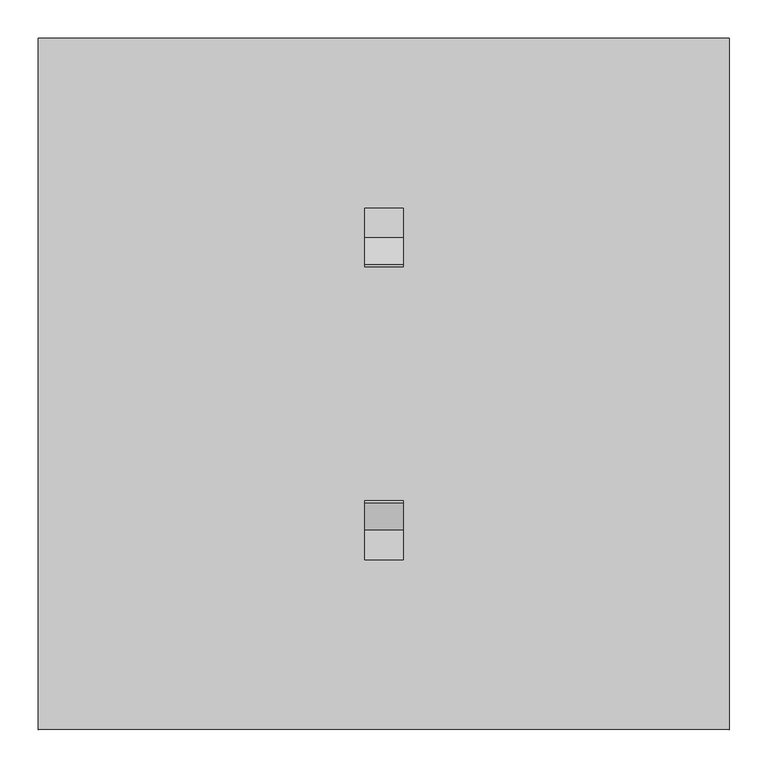
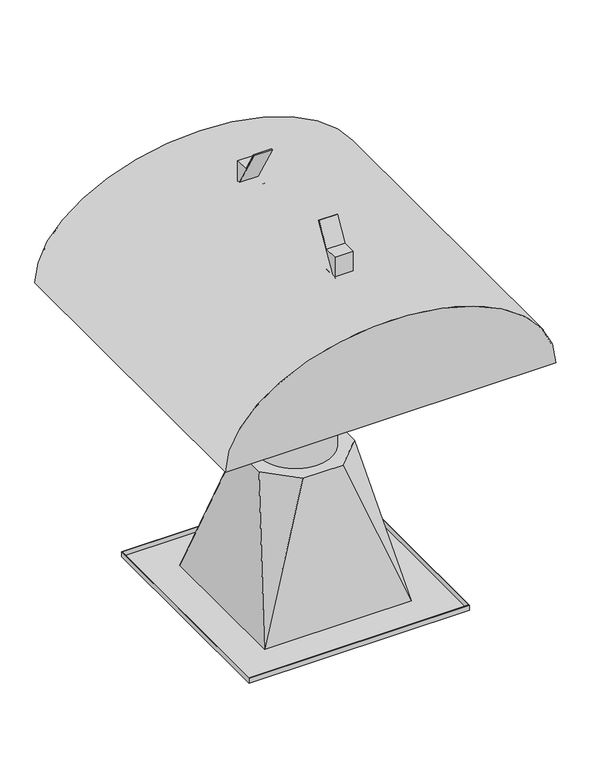
"""IFC4 building model written with IfcOpenShell, lengths in millimetres: proxy geometry, ВЕЗА_ВКОП : ВКОПО-040-Н-00."""

from ifc_helpers import new_model, si_unit, point, frame, frame_2d, origin, place, context, project, spatial, polyline, circle_curve, ellipse_curve, trimmed, segment, composite_curve, outline, extrude, faceted_brep, source, transform, mapped, element, save
from ifc_brep_helpers import plane_surface, cylinder_surface, revolved_surface, extruded_surface, advanced_brep


def mechanical_equipment_59a7846b(model_context):
    return source(origin(), model_context, "Body", "SolidModel", [
        extrude(outline(composite_curve([segment(trimmed(circle_curve(frame_2d((0.0, -15.0)), 15.0), [point((0.0, -30.0))], [point((0.0, 0.0))], False, "CARTESIAN"), True, "CONTINUOUS"), segment(trimmed(circle_curve(frame_2d((0.0, -15.0)), 15.0), [point((0.0, 0.0))], [point((0.0, -30.0))], False, "CARTESIAN"), True, "CONTINUOUS")], self_intersect=False), holes=[composite_curve([segment(trimmed(circle_curve(frame_2d((0.0, -15.0)), 8.0), [point((0.0, -23.0))], [point((0.0, -7.0))], True, "CARTESIAN"), True, "CONTINUOUS"), segment(trimmed(circle_curve(frame_2d((0.0, -15.0)), 8.0), [point((0.0, -7.0))], [point((0.0, -23.0))], True, "CARTESIAN"), True, "CONTINUOUS")], self_intersect=False)]), frame((119.501046, -59.3969696, 580.0), z_axis=(0.7071067811865491, 0.7071067811865459, 0.0), x_axis=(-0.7071067811865459, 0.7071067811865491, 0.0)), (0.0, 0.0, 1.0), 10.0),
        extrude(outline(composite_curve([segment(trimmed(circle_curve(frame_2d((0.0, -15.0)), 15.0), [point((0.0, -30.0))], [point((0.0, 0.0))], False, "CARTESIAN"), True, "CONTINUOUS"), segment(trimmed(circle_curve(frame_2d((0.0, -15.0)), 15.0), [point((0.0, 0.0))], [point((0.0, -30.0))], False, "CARTESIAN"), True, "CONTINUOUS")], self_intersect=False), holes=[composite_curve([segment(trimmed(circle_curve(frame_2d((0.0, -15.0)), 8.0), [point((0.0, -23.0))], [point((0.0, -7.0))], True, "CARTESIAN"), True, "CONTINUOUS"), segment(trimmed(circle_curve(frame_2d((0.0, -15.0)), 8.0), [point((0.0, -7.0))], [point((0.0, -23.0))], True, "CARTESIAN"), True, "CONTINUOUS")], self_intersect=False)]), frame((52.3259018, -126.5721138, 580.0), z_axis=(0.7071067811865491, 0.7071067811865459, 0.0), x_axis=(-0.7071067811865459, 0.7071067811865491, 0.0)), (0.0, 0.0, 1.0), 10.0),
        extrude(outline(composite_curve([segment(trimmed(circle_curve(frame_2d((89.4490078, -89.4490078)), 15.0), [point((100.0556095, -78.8424061))], [point((78.8424061, -100.0556095))], False, "CARTESIAN"), True, "CONTINUOUS"), segment(trimmed(circle_curve(frame_2d((89.4490078, -89.4490078)), 15.0), [point((78.8424061, -100.0556095))], [point((100.0556095, -78.8424061))], False, "CARTESIAN"), True, "CONTINUOUS")], self_intersect=False), holes=[composite_curve([segment(trimmed(circle_curve(frame_2d((89.4490078, -89.4490078)), 8.0), [point((95.1058621, -83.7921536))], [point((83.7921536, -95.1058621))], True, "CARTESIAN"), True, "CONTINUOUS"), segment(trimmed(circle_curve(frame_2d((89.4490078, -89.4490078)), 8.0), [point((83.7921536, -95.1058621))], [point((95.1058621, -83.7921536))], True, "CARTESIAN"), True, "CONTINUOUS")], self_intersect=False)]), frame((0.0, 0.0, 512.5), z_axis=(0.0, 0.0, 1.0), x_axis=(1.0, 0.0, 0.0)), (0.0, 0.0, 1.0), 10.0),
        extrude(outline(composite_curve([segment(trimmed(circle_curve(frame_2d((89.4490078, -89.4490078)), 15.0), [point((100.0556095, -78.8424061))], [point((78.8424061, -100.0556095))], False, "CARTESIAN"), True, "CONTINUOUS"), segment(trimmed(circle_curve(frame_2d((89.4490078, -89.4490078)), 15.0), [point((78.8424061, -100.0556095))], [point((100.0556095, -78.8424061))], False, "CARTESIAN"), True, "CONTINUOUS")], self_intersect=False), holes=[composite_curve([segment(trimmed(circle_curve(frame_2d((89.4490078, -89.4490078)), 8.0), [point((95.1058621, -83.7921536))], [point((83.7921536, -95.1058621))], True, "CARTESIAN"), True, "CONTINUOUS"), segment(trimmed(circle_curve(frame_2d((89.4490078, -89.4490078)), 8.0), [point((83.7921536, -95.1058621))], [point((95.1058621, -83.7921536))], True, "CARTESIAN"), True, "CONTINUOUS")], self_intersect=False)]), frame((0.0, 0.0, 607.5), z_axis=(0.0, 0.0, 1.0), x_axis=(1.0, 0.0, 0.0)), (0.0, 0.0, 1.0), 10.0),
        extrude(outline(polyline([(137.1787156, -77.0746391), (77.0746391, -137.1787156), (41.7193001, -101.8233765), (101.8233765, -41.7193001), (137.1787156, -77.0746391)])), frame((0.0, 0.0, 522.5), z_axis=(0.0, 0.0, 1.0), x_axis=(1.0, 0.0, 0.0)), (0.0, 0.0, 1.0), 85.0),
        extrude(outline(polyline([(190.7885358, 1086.3333333), (229.0846729, 1086.3333333), (229.0846729, 1030.0), (219.8766872, 1030.0), (152.3533268, 1146.953891), (154.9302621, 1148.4416853), (190.7885358, 1086.3333333)])), frame((-25.0, 0.0, 0.0), z_axis=(1.0, 0.0, 0.0), x_axis=(0.0, 1.0, 0.0)), (0.0, 0.0, 1.0), 50.0),
        extrude(outline(polyline([(189.0846729, 730.0), (189.0846729, 1028.0), (229.0846729, 1028.0), (448.0, 928.6666667), (448.0, 829.3333333), (229.0846729, 730.0), (189.0846729, 730.0)]), holes=[polyline([(194.0846729, 735.0), (228.0033477, 735.0), (443.0, 832.5552256), (443.0, 925.4447744), (228.0033477, 1023.0), (194.0846729, 1023.0), (194.0846729, 735.0)])]), frame((-25.0, 0.0, 0.0), z_axis=(1.0, 0.0, 0.0), x_axis=(0.0, 1.0, 0.0)), (0.0, 0.0, 1.0), 50.0),
        extrude(outline(polyline([(-190.7885358, 1086.3333333), (-154.9302621, 1148.4416853), (-152.3533268, 1146.953891), (-219.8766872, 1030.0), (-229.0846729, 1030.0), (-229.0846729, 1086.3333333), (-190.7885358, 1086.3333333)])), frame((-25.0, 0.0, 0.0), z_axis=(1.0, 0.0, 0.0), x_axis=(0.0, 1.0, 0.0)), (0.0, 0.0, 1.0), 50.0),
        extrude(outline(polyline([(-189.0846729, 730.0), (-229.0846729, 730.0), (-448.0, 829.3333333), (-448.0, 928.6666667), (-229.0846729, 1028.0), (-189.0846729, 1028.0), (-189.0846729, 730.0)]), holes=[polyline([(-194.0846729, 735.0), (-194.0846729, 1023.0), (-228.0033477, 1023.0), (-443.0, 925.4447744), (-443.0, 832.5552256), (-228.0033477, 735.0), (-194.0846729, 735.0)])]), frame((-25.0, 0.0, 0.0), z_axis=(1.0, 0.0, 0.0), x_axis=(0.0, 1.0, 0.0)), (0.0, 0.0, 1.0), 50.0),
        faceted_brep([(130.0, 53.8477631, 400.0), (53.8477631, 130.0, 400.0), (-53.8477631, 130.0, 400.0), (-130.0, 53.8477631, 400.0), (-130.0, -53.8477631, 400.0), (-53.8477631, -130.0, 400.0), (53.8477631, -130.0, 400.0), (130.0, -53.8477631, 400.0), (200.0, 200.0, 0.0), (200.0, -200.0, 0.0), (-200.0, -200.0, 0.0), (-200.0, 200.0, 0.0)], [[[0, 1, 2, 3, 4, 5, 6, 7]], [[8, 9, 10, 11]], [[1, 0, 8]], [[8, 11, 2, 1]], [[3, 2, 11]], [[11, 10, 4, 3]], [[5, 4, 10]], [[10, 9, 6, 5]], [[7, 6, 9]], [[9, 8, 0, 7]]]),
        advanced_brep(
        [(450.0, -450.0, 750.0), (-450.0, -450.0, 750.0), (450.0, 450.0, 750.0), (-450.0, 450.0, 750.0), (-448.0, -448.0, 750.0), (448.0, -448.0, 750.0), (448.0, 448.0, 750.0), (-448.0, 448.0, 750.0)],
        [
            (0, 1, ellipse_curve(frame((0.0, -450.0, 750.0), z_axis=(0.0, -1.0, 0.0), x_axis=(-1.0, 0.0, 0.0)), 450.0, 280.0)),
            (1, 0),
            (2, 3),
            (3, 2, ellipse_curve(frame((0.0, 450.0, 750.0), z_axis=(0.0, 1.0, 0.0), x_axis=(-1.0, 0.0, 0.0)), 450.0, 280.0)),
            (0, 2),
            (3, 1),
            (4, 5),
            (5, 6),
            (6, 7),
            (7, 4),
            (4, 5, ellipse_curve(frame((0.0, -448.0, 750.0), z_axis=(0.0, 1.0, 0.0), x_axis=(-1.0, 0.0, 0.0)), 448.0, 278.0)),
            (6, 7, ellipse_curve(frame((0.0, 448.0, 750.0), z_axis=(0.0, -1.0, 0.0), x_axis=(-1.0, 0.0, 0.0)), 448.0, 278.0)),
        ],
        [
            plane_surface(frame((-450.0, -450.0, 750.0), z_axis=(0.0, -1.0, 0.0), x_axis=(0.0, 0.0, -1.0))),
            plane_surface(frame((-450.0, 450.0, 750.0), z_axis=(0.0, 1.0, 0.0), x_axis=(0.0, 0.0, 1.0))),
            extruded_surface(trimmed(ellipse_curve(frame((0.0, 1350.0, 750.0), z_axis=(0.0, -1.0, 0.0), x_axis=(-1.0, 0.0, 0.0)), 450.0, 280.0), [point((450.0, 1350.0, 750.0))], [point((-450.0, 1350.0, 750.0))], True, "CARTESIAN"), (0.0, -900.0, 0.0), 900.0),
            plane_surface(frame((-450.0, -450.0, 750.0), z_axis=(0.0, 0.0, -1.0), x_axis=(0.0, 1.0, 0.0))),
            plane_surface(frame((-448.0, -448.0, 750.0), z_axis=(0.0, 1.0, 0.0), x_axis=(0.0, 0.0, -1.0))),
            plane_surface(frame((-448.0, 448.0, 750.0), z_axis=(0.0, -1.0, 0.0), x_axis=(0.0, 0.0, 1.0))),
            extruded_surface(trimmed(ellipse_curve(frame((0.0, 448.0, 750.0), z_axis=(0.0, -1.0, 0.0), x_axis=(-1.0, 0.0, 0.0)), 448.0, 278.0), [point((448.0, 448.0, 750.0))], [point((-448.0, 448.0, 750.0))], True, "CARTESIAN"), (0.0, 896.0, 0.0), 896.0),
        ],
        [
            (0, [[1, 2]]),
            (1, [[3, 4]]),
            (2, [[-1, 5, -4, 6]]),
            (3, [[-2, -6, -3, -5], [7, 8, 9, 10]]),
            (4, [[11, -7]]),
            (5, [[12, -9]]),
            (6, [[-11, -10, -12, -8]]),
        ],
    ),
        advanced_brep(
        [(130.0, 0.0, 730.0), (-130.0, 0.0, 730.0), (-45.0, 0.0, 730.0), (45.0, 0.0, 730.0), (100.0, 0.0, 686.5584821), (-100.0, 0.0, 686.5584821), (100.0, 0.0, 400.0), (-100.0, 0.0, 400.0), (0.0, 0.0, 400.0), (-45.0, 0.0, 750.0), (45.0, 0.0, 750.0)],
        [
            (0, 1, circle_curve(frame((0.0, 0.0, 730.0), z_axis=(0.0, 0.0, 1.0), x_axis=(-1.0, 0.0, 0.0)), 130.0)),
            (1, 2),
            (2, 3, circle_curve(frame((0.0, 0.0, 730.0), z_axis=(0.0, 0.0, -1.0), x_axis=(-1.0, 0.0, 0.0)), 45.0)),
            (3, 0),
            (1, 0, circle_curve(frame((0.0, 0.0, 730.0), z_axis=(0.0, 0.0, 1.0), x_axis=(-1.0, 0.0, 0.0)), 130.0)),
            (3, 2, circle_curve(frame((0.0, 0.0, 730.0), z_axis=(0.0, 0.0, -1.0), x_axis=(-1.0, 0.0, 0.0)), 45.0)),
            (0, 4, circle_curve(frame((151.2012649, 0.0, 683.2792411), z_axis=(0.0, -1.0, 0.0), x_axis=(-1.0, 0.0, 0.0)), 51.3061687)),
            (4, 5, circle_curve(frame((0.0, 0.0, 686.5584821), z_axis=(0.0, 0.0, 1.0), x_axis=(-1.0, 0.0, 0.0)), 100.0)),
            (5, 1, circle_curve(frame((-151.2012649, 0.0, 683.2792411), z_axis=(0.0, -1.0, 0.0), x_axis=(1.0, 0.0, 0.0)), 51.3061687)),
            (5, 4, circle_curve(frame((0.0, 0.0, 686.5584821), z_axis=(0.0, 0.0, 1.0), x_axis=(-1.0, 0.0, 0.0)), 100.0)),
            (4, 6),
            (6, 7, circle_curve(frame((0.0, 0.0, 400.0), z_axis=(0.0, 0.0, 1.0), x_axis=(-1.0, 0.0, 0.0)), 100.0)),
            (7, 5),
            (7, 6, circle_curve(frame((0.0, 0.0, 400.0), z_axis=(0.0, 0.0, 1.0), x_axis=(-1.0, 0.0, 0.0)), 100.0)),
            (6, 8),
            (8, 7),
            (2, 9),
            (9, 10, circle_curve(frame((0.0, 0.0, 750.0), z_axis=(0.0, 0.0, -1.0), x_axis=(-1.0, 0.0, 0.0)), 45.0)),
            (10, 3),
            (10, 9, circle_curve(frame((0.0, 0.0, 750.0), z_axis=(0.0, 0.0, -1.0), x_axis=(-1.0, 0.0, 0.0)), 45.0)),
        ],
        [
            plane_surface(frame((0.0, 0.0, 730.0), z_axis=(0.0, 0.0, 1.0), x_axis=(-1.0, 0.0, 0.0))),
            revolved_surface(trimmed(ellipse_curve(frame((-151.2012649, 0.0, 683.2792411), z_axis=(0.0, 1.0, 0.0), x_axis=(1.0, 0.0, 0.0)), 51.3061687, 51.3061687), [point((-130.0, 0.0, 730.0))], [point((-100.0, 0.0, 686.5584821))], True, "CARTESIAN"), (0.0, 0.0, 710.0), (0.0, 0.0, -1.0)),
            cylinder_surface(frame((0.0, 0.0, 710.0), z_axis=(0.0, 0.0, -1.0), x_axis=(-1.0, 0.0, 0.0)), 100.0),
            plane_surface(frame((0.0, 0.0, 400.0), z_axis=(0.0, 0.0, -1.0), x_axis=(-1.0, 0.0, 0.0))),
            cylinder_surface(frame((0.0, 0.0, 710.0), z_axis=(0.0, 0.0, -1.0), x_axis=(-1.0, 0.0, 0.0)), 45.0),
            plane_surface(frame((-448.0, -448.0, 750.0), z_axis=(0.0, 0.0, 1.0), x_axis=(0.0, 1.0, 0.0))),
        ],
        [
            (0, [[1, 2, 3, 4]]),
            (0, [[-2, 5, -4, 6]]),
            (1, [[-1, 7, 8, 9]]),
            (1, [[-5, -9, 10, -7]]),
            (2, [[-8, 11, 12, 13]]),
            (2, [[-10, -13, 14, -11]]),
            (3, [[-12, 15, 16]]),
            (3, [[-14, -16, -15]]),
            (4, [[-3, 17, 18, 19]]),
            (4, [[-6, -19, 20, -17]]),
            (5, [[-18, -20]]),
        ],
    ),
        faceted_brep([(-200.0, -200.0, 0.0), (-200.0, -200.0, 1.5), (200.0, -200.0, 1.5), (200.0, -200.0, 0.0), (-300.0, -300.0, 15.0), (-300.0, -300.0, 0.0), (300.0, -300.0, 0.0), (300.0, -300.0, 15.0), (-298.5, -298.5, 1.5), (-298.5, -298.5, 15.0), (298.5, -298.5, 15.0), (298.5, -298.5, 1.5), (200.0, 200.0, 1.5), (200.0, 200.0, 0.0), (300.0, 300.0, 0.0), (300.0, 300.0, 15.0), (298.5, 298.5, 15.0), (298.5, 298.5, 1.5), (-200.0, 200.0, 1.5), (-200.0, 200.0, 0.0), (-300.0, 300.0, 0.0), (-300.0, 300.0, 15.0), (-298.5, 298.5, 15.0), (-298.5, 298.5, 1.5)], [[[0, 1, 2, 3]], [[4, 5, 6, 7]], [[8, 9, 10, 11]], [[3, 2, 12, 13]], [[7, 6, 14, 15]], [[11, 10, 16, 17]], [[13, 12, 18, 19]], [[15, 14, 20, 21]], [[17, 16, 22, 23]], [[19, 18, 1, 0]], [[5, 20, 14, 6], [3, 13, 19, 0]], [[21, 20, 5, 4]], [[7, 15, 21, 4], [9, 22, 16, 10]], [[23, 22, 9, 8]], [[11, 17, 23, 8], [1, 18, 12, 2]]]),
    ])


if __name__ == "__main__":
    model = new_model("IFC4")
    model_context = context("Model", 3, world=origin())
    ifc_project = project(units=[si_unit("LENGTHUNIT", "METRE", prefix="MILLI")], contexts=[model_context])
    site = spatial("IfcSite", under=ifc_project)
    building = spatial("IfcBuilding", under=site)
    placement = place(None, origin())
    mechanical_equipment_shape = mechanical_equipment_59a7846b(model_context)
    element("IfcBuildingElementProxy", 1, Name="ВЕЗА_ВКОП : ВКОПО-040-Н-00", ObjectType="ВЕЗА_ВКОП : ВКОПО-040-Н-00", at=placement, inside=building, context=model_context, shape_type="MappedRepresentation", body=[
        mapped(mechanical_equipment_shape, transform((0.0, 0.0, 0.0), x_axis=(1.0, 0.0, 0.0), y_axis=(0.0, 1.0, 0.0), z_axis=(0.0, 0.0, 1.0))),
    ])
    save(model, "model.ifc")

# Revit data of these elements
# Type "ВЕЗА_ВКОП : ВКОПО-040-Н-00"
#   Таблица_ВКОП = "ВКОП"
#   Класс энергоэффективности электродвигателя = "IE2"
#   ВЕЗА_Контакты = "bim@veza.ru"
#   ВЕЗА_Классификатор = "79001"
#   URL = "http://www.veza.ru/upload/iblock/0e3/%D0%92%D0%9A%D0%9E%D0%9F%20%D0%B0%D0%B2%D0%B3%D1%83%D1%81%D1%82%202019%20%D1%80%D0%B5%D0%B4%D0%B0%D0%BA%D1%82%20270919-1.pdf"
#   ADSK_Примечание = ""
#   ADSK_Позиция = "1"
#   ADSK_Наименование краткое = "ВКОП"
#   ADSK_Наименование = "Агрегат крышный ВКОП 0 типоразмер 040; общепромышленного исполнения; номинальная мощность Nnon=1,1 кВт, число полюсов 2; климатическое исполение УХЛ1"
#   ADSK_Марка = "ВКОПО-040-Н-00110/2-УХЛ1 ТУ 4861-152-40149153-2010"
#   ADSK_Комплект [instance default] = ""
#   ADSK_Код изделия = ""
#   ADSK_Завод-изготовитель = "ООО \"Веза\", Россия, Москва, ИНН 505001001, info@veza.ru"
#   ADSK_Единица измерения = "компл."
#   ADSK_Дата изменения = "23.03.2020"
#   ADSK_Группирование = ""
#   ADSK_Версия семейства = "Версия 1"
#   ADSK_Версия Revit = "Revit2018"
#   Угол поворота УГО_3D [instance default] = 45°
#   Default Elevation = 1219.2 mm
#   x2 = -448 mm
#   x1 = 448 mm
#   r = 100 mm
#   H3 = 300 mm
#   H2 = 1000 mm
#   H1 = 630 mm
#   H = 400 mm
#   D = 200 mm
#   B = 900 mm
#   ADSK_Ток = 1.52778 A
#   ADSK_Свободный напор воздуха [instance default] = 0.0 Pa
#   ADSK_Расход воздуха [instance default] = 0 m³/h
#   ADSK_Размер_Ширина = 400 mm
#   ADSK_Размер_Длина [instance default] = 400 mm
#   ADSK_Потеря давления воздуха [instance default] = 0.0 Pa
#   ADSK_Полная мощность = 611.111 VA
#   ADSK_Номинальная мощность = 550 W
#   ADSK_Напряжение = 400 V
#   ADSK_Масса = 44
#   ADSK_Коэффициент мощности = 0.9
#   A2 = 260 mm
#   A1 = 600 mm
#   A = 400 mm
#   Число полюсов = 4
#   Типоразмер [instance default] = 40
#   Тип основания = 1
#   Масштаб УГО [instance default] = 100
#   ВЕЗА_Типоразмер = 40
#   ADSK_Частота вращения двигателя = 1500
#   ADSK_Частота вращения вентилятора = 1500
#   ADSK_Количество фаз числовое = 3
#   ADSK_Количество фаз = 3
#   ADSK_Материал [instance default] = ВЕЗА_сталь оцинкованная
#   ADSK_Классификация нагрузок = ОВК
#   Description = (empty or 0)
#   Manufacturer = ""
# Element 1 (IfcBuildingElementProxy, "ВЕЗА_ВКОП : ВКОПО-040-Н-00")
#   ADSK_Размер_Длина = 560 mm
#   Типоразмер = 56
#   Materials on its faces: "ВЕЗА_сталь оцинкованная", "Пластмасса коробки"
# Materials
#   "ВЕЗА_сталь оцинкованная": class "Типовые", colour RGB 120 120 120, transparency 0, Cost = 0
#   "Пластмасса коробки": class "Типовые", colour RGB 120 120 120, transparency 0, Cost = 0
